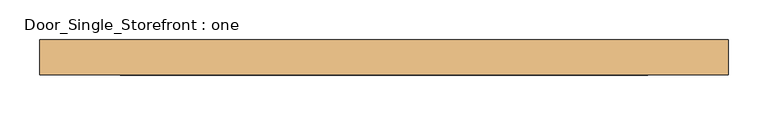
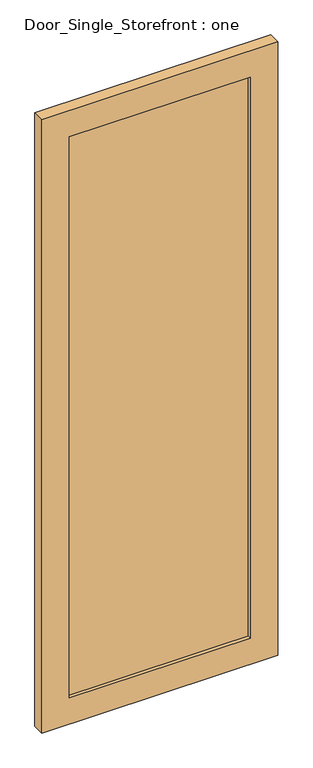
"""IFC4 building model written with IfcOpenShell, lengths in millimetres: door geometry, Door_Single_Storefront : one."""

from ifc_helpers import new_model, si_unit, frame, origin, place, context, project, spatial, polyline, outline, extrude, source, transform, mapped, element, save


def door_single_storefront_one_dd4e76e3(model_context):
    return source(origin(), model_context, "Body", "SweptSolid", [
        extrude(outline(polyline([(2387.6, -434.18125), (0.0, -434.18125), (0.0, 434.18125), (2387.6, 434.18125), (2387.6, -434.18125)]), holes=[polyline([(101.6, 332.58125), (101.6, -332.58125), (2286.0, -332.58125), (2286.0, 332.58125), (101.6, 332.58125)])]), frame((0.0, -25.4, 0.0), z_axis=(0.0, 1.0, 0.0), x_axis=(0.0, 0.0, 1.0)), (0.0, 0.0, 1.0), 44.45),
        extrude(outline(polyline([(332.58125, 6.35), (332.58125, -12.7), (-332.58125, -12.7), (-332.58125, 6.35), (332.58125, 6.35)])), frame((0.0, 0.0, 101.6), z_axis=(0.0, 0.0, 1.0), x_axis=(1.0, 0.0, 0.0)), (0.0, 0.0, 1.0), 2184.4),
    ])


if __name__ == "__main__":
    model = new_model("IFC4")
    model_context = context("Model", 3, world=origin())
    ifc_project = project(units=[si_unit("LENGTHUNIT", "METRE", prefix="MILLI")], contexts=[model_context])
    site = spatial("IfcSite", under=ifc_project)
    building = spatial("IfcBuilding", under=site)
    placement = place(None, origin())
    door_single_storefront_one_shape = door_single_storefront_one_dd4e76e3(model_context)
    element("IfcDoor", 1, ObjectType="Door_Single_Storefront : one", at=placement, inside=building, context=model_context, shape_type="MappedRepresentation", body=[
        mapped(door_single_storefront_one_shape, transform((0.0, 0.0, 0.0), x_axis=(1.0, 0.0, 0.0), y_axis=(0.0, 1.0, 0.0), z_axis=(0.0, 0.0, 1.0))),
    ])
    save(model, "model.ifc")

# Revit data of these elements
# Type "Door_Single_Storefront : one"
#   Type Mark = "27"
#   Analytic Construction = "<None>"
#   Stile_Width = 0' - 4"
#   Door_Thickness = 0' - 1 3/4"
#   Door_Offset = 0' - 1"
#   Glass_Material = Glass
#   Frame_Material = Aluminum
#   Function = (empty or 0)
# Element 1 (IfcDoor, "Door_Single_Storefront : one")
#   Materials on its faces: "Aluminum", "Glass"
# Materials
#   "Glass": class "Glass", colour RGB 142 168 196, transparency 0.75, Description = "Soda Lime Glass", Cost = 0
#   "Aluminum": class "Metal", colour RGB 226 226 226, transparency 0, Description = "Aluminum 6061", Cost = 0
